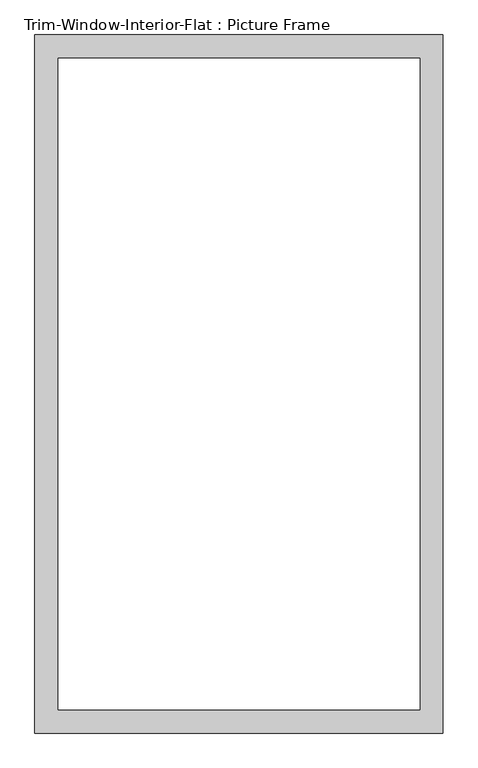
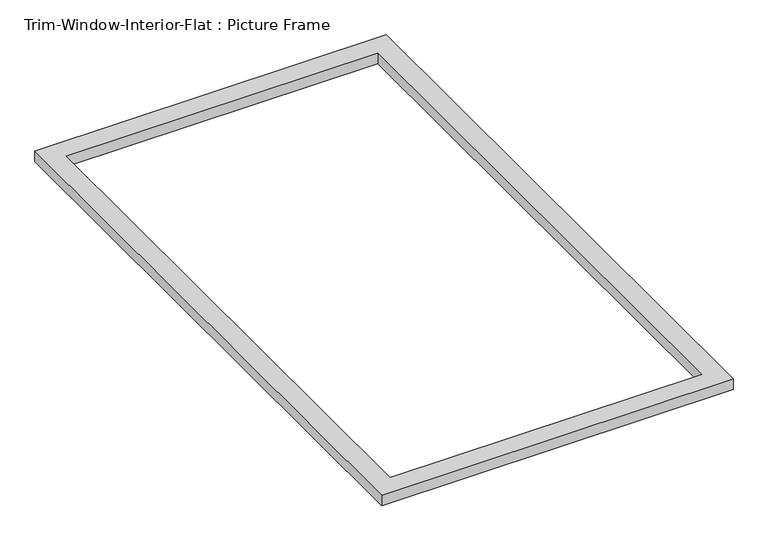
"""IFC4 building model written with IfcOpenShell, lengths in millimetres: proxy geometry, Trim-Window-Interior-Flat : Picture Frame."""

import ifcopenshell
import ifcopenshell.guid

model = None  # the IFC model being written
_history = None  # IfcOwnerHistory: only IFC2X3 demands one
_inside = {}  # id of a spatial element -> (the spatial element, [elements in it])
_under = {}  # id of a project, library or spatial element -> (it, [spatial elements below it])
_declared = {}  # id of a project -> (the project, [libraries it declares])
_typed = {}  # id of a type object -> (the type object, [elements of that type])
_made_of = {}  # id of a material, layer set ... -> (it, [elements and type objects made of it])


def new_model(schema):
    """Start an empty IFC model of exactly this schema.

    Asked for "IFC4X3", IfcOpenShell would pick the latest addendum, in which some entities
    have other attributes; the version numbers below select the first issue.
    IFC2X3 requires an IfcOwnerHistory on every rooted entity: one is made here for all.
    """
    global model, _history
    if schema == "IFC4X3":
        model = ifcopenshell.file(schema_version=(4, 3, 0, 0))
    else:
        model = ifcopenshell.file(schema=schema)
    _inside.clear()
    _under.clear()
    _declared.clear()
    _typed.clear()
    _made_of.clear()
    _history = None
    if model.schema == "IFC2X3":
        org = make("IfcOrganization", Name="unknown")
        user = make(
            "IfcPersonAndOrganization",
            ThePerson=make("IfcPerson", FamilyName="unknown"),
            TheOrganization=org,
        )
        app = make(
            "IfcApplication",
            ApplicationDeveloper=org,
            Version="unknown",
            ApplicationFullName="unknown",
            ApplicationIdentifier="unknown",
        )
        _history = make(
            "IfcOwnerHistory",
            OwningUser=user,
            OwningApplication=app,
            ChangeAction="ADDED",
            CreationDate=0,
        )
    return model


def make(cls, **values):
    """One entity of the class cls with the attributes given. An attribute that is None is left unset."""
    return model.create_entity(
        cls, **{name: value for name, value in values.items() if value is not None}
    )


def rooted(cls, **values):
    """An entity with a GlobalId (a new one), such as an element, a storey or a relation."""
    return make(cls, GlobalId=ifcopenshell.guid.new(), OwnerHistory=_history, **values)


def si_unit(unit_type, name, prefix=None):
    """IfcSIUnit, for example si_unit("LENGTHUNIT", "METRE", prefix="MILLI")."""
    return make("IfcSIUnit", UnitType=unit_type, Prefix=prefix, Name=name)


def assignment(units):
    """IfcUnitAssignment: the units of a project."""
    return None if units is None else make("IfcUnitAssignment", Units=units)


def point(xyz):
    """IfcCartesianPoint."""
    return None if xyz is None else make("IfcCartesianPoint", Coordinates=xyz)


def direction(xyz):
    """IfcDirection."""
    return None if xyz is None else make("IfcDirection", DirectionRatios=xyz)


def frame(location, z_axis=None, x_axis=None):
    """IfcAxis2Placement3D, a coordinate frame: its origin and axes. An axis left out is left unset."""
    return make(
        "IfcAxis2Placement3D",
        Location=point(location),
        Axis=direction(z_axis),
        RefDirection=direction(x_axis),
    )


def origin():
    """The frame at (0, 0, 0) with its axes left unset."""
    return frame((0.0, 0.0, 0.0))


def origin_with_axes():
    """The frame at (0, 0, 0) with the z axis (0, 0, 1) and the x axis (1, 0, 0) written out."""
    return frame((0.0, 0.0, 0.0), z_axis=(0.0, 0.0, 1.0), x_axis=(1.0, 0.0, 0.0))


def place(relative_to, where):
    """IfcLocalPlacement: puts the frame where relative to a parent placement (None: the world)."""
    return make(
        "IfcLocalPlacement", PlacementRelTo=relative_to, RelativePlacement=where
    )


def context(
    kind, dimensions, precision=None, world=None, true_north=None, identifier=None
):
    """IfcGeometricRepresentationContext, for example the 3D "Model" context."""
    return make(
        "IfcGeometricRepresentationContext",
        ContextIdentifier=identifier,
        ContextType=kind,
        CoordinateSpaceDimension=dimensions,
        Precision=precision,
        WorldCoordinateSystem=world,
        TrueNorth=true_north,
    )


def project(units=None, contexts=None):
    """IfcProject with its units and contexts."""
    return rooted(
        "IfcProject",
        Name="project",
        RepresentationContexts=contexts,
        UnitsInContext=assignment(units),
    )


def spatial(cls, under=None, at=None, **own):
    """A site, building, storey or space (cls), placed at a placement, below another one or the project."""
    s = rooted(cls, ObjectPlacement=at, **own)
    if under is not None:
        _under.setdefault(under.id(), (under, []))[1].append(s)
    return s


def polyline(points):
    """IfcPolyline through the points."""
    return make("IfcPolyline", Points=[point(p) for p in points])


def outline(outer, holes=None, kind="AREA"):
    """IfcArbitraryClosedProfileDef: a profile drawn as a closed curve; with holes, ...WithVoids."""
    if holes is None:
        return make("IfcArbitraryClosedProfileDef", ProfileType=kind, OuterCurve=outer)
    return make(
        "IfcArbitraryProfileDefWithVoids",
        ProfileType=kind,
        OuterCurve=outer,
        InnerCurves=holes,
    )


def extrude(swept, where, along, depth):
    """IfcExtrudedAreaSolid: the profile swept, set in the frame where, extruded along a direction by depth."""
    return make(
        "IfcExtrudedAreaSolid",
        SweptArea=swept,
        Position=where,
        ExtrudedDirection=direction(along),
        Depth=depth,
    )


def shape(context_of_items, identifier, shape_type, items):
    """IfcShapeRepresentation: the items that make up one representation, for example the "Body"."""
    return make(
        "IfcShapeRepresentation",
        ContextOfItems=context_of_items,
        RepresentationIdentifier=identifier,
        RepresentationType=shape_type,
        Items=items,
    )


def source(mapping_origin, context_of_items, identifier, shape_type, items):
    """IfcRepresentationMap: a shape defined once, which mapped items show again and again."""
    return make(
        "IfcRepresentationMap",
        MappingOrigin=mapping_origin,
        MappedRepresentation=shape(context_of_items, identifier, shape_type, items),
    )


def transform(
    local_origin,
    x_axis=None,
    y_axis=None,
    z_axis=None,
    scale=None,
    scale2=None,
    scale3=None,
    uniform=True,
):
    """IfcCartesianTransformationOperator3D, or its non-uniform kind. x_axis, y_axis, z_axis: its Axis1, 2, 3."""
    if uniform:
        return make(
            "IfcCartesianTransformationOperator3D",
            Axis1=direction(x_axis),
            Axis2=direction(y_axis),
            LocalOrigin=point(local_origin),
            Scale=scale,
            Axis3=direction(z_axis),
        )
    return make(
        "IfcCartesianTransformationOperator3DnonUniform",
        Axis1=direction(x_axis),
        Axis2=direction(y_axis),
        LocalOrigin=point(local_origin),
        Scale=scale,
        Axis3=direction(z_axis),
        Scale2=scale2,
        Scale3=scale3,
    )


def mapped(mapping_source, mapping_target):
    """IfcMappedItem: shows the shape of a source again, moved by a transform."""
    return make(
        "IfcMappedItem", MappingSource=mapping_source, MappingTarget=mapping_target
    )


def made_of(thing, what):
    """Note that an element or type object is made of a material, layer set ...; save() writes the relation."""
    if what is not None:
        _made_of.setdefault(what.id(), (what, []))[1].append(thing)
    return thing


def element(
    cls,
    number,
    at=None,
    inside=None,
    cuts=None,
    type_object=None,
    material=None,
    context=None,
    identifier="Body",
    shape_type=None,
    held_by="IfcProductDefinitionShape",
    body=None,
    shapes=None,
    **own,
):
    """One element of the class cls, such as IfcWall. Its Tag is "e" and its number.

    at: its placement. inside: the storey or other place that contains it. cuts: it is an
    opening in that element (IfcRelVoidsElement). A single representation is given by context,
    identifier, shape_type and body (its items); several are given by shapes. held_by: the class
    of the entity that holds the representations. save() writes the other relations.
    """
    e = rooted(cls, Tag="e%d" % number, ObjectPlacement=at, **own)
    if body is not None:
        shapes = [shape(context, identifier, shape_type, body)]
    if shapes is not None:
        e.Representation = make(held_by, Representations=shapes)
    if inside is not None:
        _inside.setdefault(inside.id(), (inside, []))[1].append(e)
    if cuts is not None:
        rooted(
            "IfcRelVoidsElement", RelatingBuildingElement=cuts, RelatedOpeningElement=e
        )
    if type_object is not None:
        _typed.setdefault(type_object.id(), (type_object, []))[1].append(e)
    return made_of(e, material)


def aggregate(whole, parts):
    """IfcRelAggregates: a whole, such as a stair, and the parts it consists of."""
    return rooted("IfcRelAggregates", RelatingObject=whole, RelatedObjects=parts)


def save(model, path):
    """Write the relations noted so far, then the file.

    IfcRelAggregates (storeys below a building ...), IfcRelContainedInSpatialStructure (elements
    in a storey), IfcRelDefinesByType, IfcRelAssociatesMaterial and IfcRelDeclares: one each for
    every whole, place, type object, material and project.
    """
    for whole, parts in _under.values():
        aggregate(whole, parts)
    for where, things in _inside.values():
        rooted(
            "IfcRelContainedInSpatialStructure",
            RelatedElements=things,
            RelatingStructure=where,
        )
    for kind, things in _typed.values():
        rooted("IfcRelDefinesByType", RelatedObjects=things, RelatingType=kind)
    for what, things in _made_of.values():
        rooted("IfcRelAssociatesMaterial", RelatedObjects=things, RelatingMaterial=what)
    for by, libraries in _declared.values():
        rooted("IfcRelDeclares", RelatingContext=by, RelatedDefinitions=libraries)
    model.write(path)


def trim_window_interior_flat_picture_frame_cf830d55(model_context):
    return source(origin(), model_context, "Body", "SweptSolid", [
        extrude(outline(polyline([(501.65, -44.45), (-501.65, -44.45), (-501.65, 1670.05), (501.65, 1670.05), (501.65, -44.45)]), holes=[polyline([(444.5, 12.7), (444.5, 1612.9), (-444.5, 1612.9), (-444.5, 12.7), (444.5, 12.7)])]), origin_with_axes(), (0.0, 0.0, 1.0), 31.75),
    ])


if __name__ == "__main__":
    model = new_model("IFC4")
    model_context = context("Model", 3, world=origin())
    ifc_project = project(units=[si_unit("LENGTHUNIT", "METRE", prefix="MILLI")], contexts=[model_context])
    site = spatial("IfcSite", under=ifc_project)
    building = spatial("IfcBuilding", under=site)
    placement = place(None, origin())
    trim_window_interior_flat_picture_frame_shape = trim_window_interior_flat_picture_frame_cf830d55(model_context)
    element("IfcBuildingElementProxy", 1, Name="Trim-Window-Interior-Flat : Picture Frame", ObjectType="Trim-Window-Interior-Flat : Picture Frame", at=placement, inside=building, context=model_context, shape_type="MappedRepresentation", body=[
        mapped(trim_window_interior_flat_picture_frame_shape, transform((0.0, 0.0, 0.0), x_axis=(1.0, 0.0, 0.0), y_axis=(0.0, 1.0, 0.0), z_axis=(0.0, 0.0, 1.0))),
    ])
    save(model, "model.ifc")

# Revit data of these elements
# Type "Trim-Window-Interior-Flat : Picture Frame"
#   Trim Thickness_Picture Frame = 0' - 1 1/4"
#   Trim Width = 0' - 2 1/4"
#   Trim Thickness_with Sill = 0' - 0 3/4"
#   Sill Thickness = 0' - 1 1/4"
#   Opening Width [instance default] = 2' - 0"
#   Opening Height [instance default] = 3' - 0"
#   Default Elevation = 4' - 0"
#   Sill = no
#   Picture Frame = yes
#   Trim Material [instance default] = none
# Element 1 (IfcBuildingElementProxy, "Trim-Window-Interior-Flat : Picture Frame")
#   Opening Width = 3' - 0"
#   Opening Height = 5' - 4"
#   Trim Material = Wood - Stained
#   Materials on its faces: "Wood - Stained"
# Materials
#   "Wood - Stained": class "Wood", colour RGB 224 178 126, transparency 0, Cost = 0
